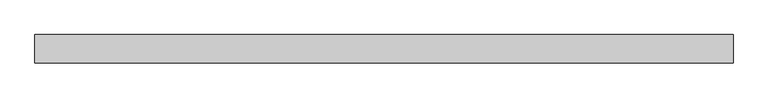
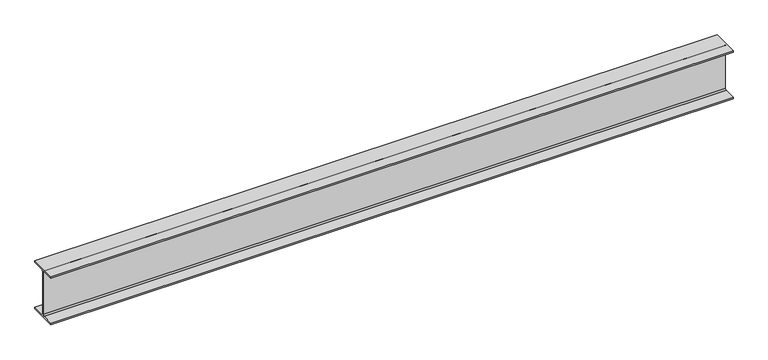
"""IFC4 building model written with IfcOpenShell, lengths in millimetres: beam geometry, Old_Steel Beam_H-KSD3502 : H_SB_ASB_H-200×200x8x12."""

from ifc_helpers import new_model, si_unit, point, frame, frame_2d, origin, place, context, project, spatial, polyline, circle_curve, trimmed, segment, composite_curve, outline, extrude, source, transform, mapped, element, save


def beam_d9134230(model_context):
    return source(origin(), model_context, "Body", "SweptSolid", [
        extrude(outline(composite_curve([segment(polyline([(82.5, -141.5), (82.5, -151.7), (-82.5, -151.7), (-82.5, -141.5), (-11.9, -141.5)]), True, "CONTINUOUS"), segment(trimmed(circle_curve(frame_2d((-11.9, -132.6)), 8.9), [point((-11.9, -141.5))], [point((-3.0, -132.6))], True, "CARTESIAN"), True, "CONTINUOUS"), segment(polyline([(-3.0, -132.6), (-3.0, 132.6)]), True, "CONTINUOUS"), segment(trimmed(circle_curve(frame_2d((-11.9, 132.6)), 8.9), [point((-3.0, 132.6))], [point((-11.9, 141.5))], True, "CARTESIAN"), True, "CONTINUOUS"), segment(polyline([(-11.9, 141.5), (-82.5, 141.5), (-82.5, 151.7), (82.5, 151.7), (82.5, 141.5), (11.9, 141.5)]), True, "CONTINUOUS"), segment(trimmed(circle_curve(frame_2d((11.9, 132.6)), 8.9), [point((11.9, 141.5))], [point((3.0, 132.6))], True, "CARTESIAN"), True, "CONTINUOUS"), segment(polyline([(3.0, 132.6), (3.0, -132.6)]), True, "CONTINUOUS"), segment(trimmed(circle_curve(frame_2d((11.9, -132.6)), 8.9), [point((3.0, -132.6))], [point((11.9, -141.5))], True, "CARTESIAN"), True, "CONTINUOUS"), segment(polyline([(11.9, -141.5), (82.5, -141.5)]), True, "CONTINUOUS")], self_intersect=False)), frame((-2035.0333333, 0.0, 0.0), z_axis=(1.0, 0.0, 0.0), x_axis=(0.0, 1.0, 0.0)), (0.0, 0.0, 1.0), 4070.0666667),
    ])


if __name__ == "__main__":
    model = new_model("IFC4")
    model_context = context("Model", 3, world=origin())
    ifc_project = project(units=[si_unit("LENGTHUNIT", "METRE", prefix="MILLI")], contexts=[model_context])
    site = spatial("IfcSite", under=ifc_project)
    building = spatial("IfcBuilding", under=site)
    placement = place(None, origin())
    beam_shape = beam_d9134230(model_context)
    element("IfcBeam", 1, ObjectType="Old_Steel Beam_H-KSD3502 : H_SB_ASB_H-200×200x8x12", at=placement, inside=building, context=model_context, shape_type="MappedRepresentation", body=[
        mapped(beam_shape, transform((0.0, 0.0, 0.0), x_axis=(1.0, 0.0, 0.0), y_axis=(0.0, 1.0, 0.0), z_axis=(0.0, 0.0, 1.0))),
    ])
    save(model, "model.ifc")

# Revit data of these elements
# Type "Old_Steel Beam_H-KSD3502 : H_SB_ASB_H-200×200x8x12"
#   Width = 20.0 cm
#   Web Thickness = 0.8 cm
#   Web Fillet = 1.3 cm
#   Warping Constant = 141376.0 cm⁶
#   Torsional Moment of Inertia = 26.2485 cm⁴
#   Torsional Modulus = 1.0 cm³
#   Section Area = 63.53 cm²
#   Plastic Modulus weak axis = 244.0 cm³
#   Plastic Modulus strong axis = 525.0 cm³
#   Perimeter = 1.16 m²/m
#   Nominal Weight = 49.90 kgf/m
#   Moment of Inertia weak axis = 1600.00 cm⁴
#   Moment of Inertia strong axis = 4720.00 cm⁴
#   Height = 20.0 cm
#   Flange Thickness = 1.2 cm
#   Elastic Modulus weak axis = 160.0 cm³
#   Elastic Modulus strong axis = 472.0 cm³
#   Centroid Vertical = 10.0 cm
#   Centroid Horizontal = 10.0 cm
#   Length [instance default] = 1.5240 m
#   Structural Material [instance default] = Steel, 45-345
#   Assembly Code = ""
# Element 1 (IfcBeam, "Old_Steel Beam_H-KSD3502 : H_SB_ASB_H-200×200x8x12")
#   Structural Material = none
# Materials
#   "Steel, 45-345": class "Metal", colour RGB 189 187 185, transparency 0, Description = "Steel 345 MPa", Cost = 0
